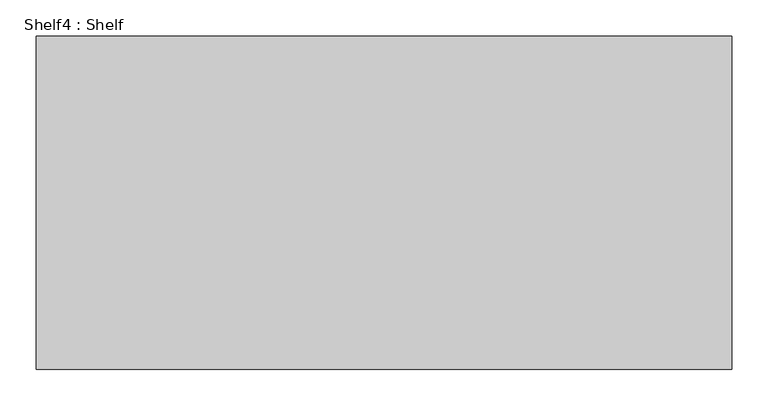
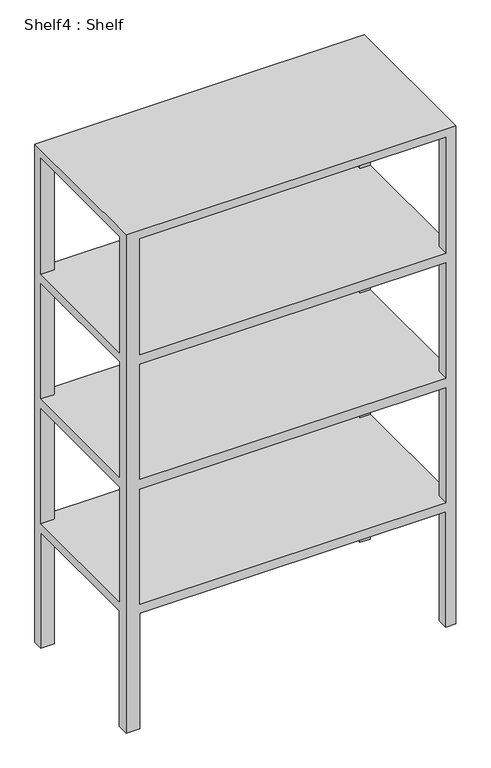
"""IFC4 building model written with IfcOpenShell, lengths in millimetres: furniture geometry, Shelf4 : Shelf."""

from ifc_helpers import new_model, si_unit, origin, place, context, project, spatial, faceted_brep, source, transform, mapped, element, save


def shelf4_shelf_8ff96b21(model_context):
    return source(origin(), model_context, "Body", "Brep", [
        faceted_brep([(14056.7001442, 2274.5615366, 1524.0), (14056.7001442, 2731.7615366, 1524.0), (13103.4798744, 2731.7615366, 1524.0), (13103.4798744, 2274.5615366, 1524.0), (14056.7001442, 2274.5615366, 0.0), (14028.3529362, 2274.5615366, 0.0), (14028.3529362, 2307.1181796, 0.0), (14056.7001442, 2307.1181796, 0.0), (14027.0281946, 2731.7615366, 0.0), (14056.7001442, 2731.7615366, 0.0), (14056.7001442, 2702.8377422, 0.0), (14027.0281946, 2702.8377422, 0.0), (13142.3001442, 2274.5615366, 0.0), (13103.4798744, 2274.5615366, 0.0), (13103.4798744, 2308.3555128, 0.0), (13142.3001442, 2308.3555128, 0.0), (13103.4798744, 2702.8377422, 0.0), (13103.4798744, 2731.7615366, 0.0), (13142.3001442, 2731.7615366, 0.0), (13142.3001442, 2702.8377422, 0.0), (13142.3001442, 2274.5615366, 353.3332002), (14028.3529362, 2274.5615366, 353.3332002), (13142.3001442, 2274.5615366, 1497.6781444), (14028.3529362, 2274.5615366, 1497.6781444), (14028.3529362, 2274.5615366, 1143.0), (13142.3001442, 2274.5615366, 1143.0), (13142.3001442, 2274.5615366, 1114.8196695), (14028.3529362, 2274.5615366, 1114.8196695), (14028.3529362, 2274.5615366, 762.0), (13142.3001442, 2274.5615366, 762.0), (13142.3001442, 2274.5615366, 731.9611947), (14028.3529362, 2274.5615366, 731.9611947), (14028.3529362, 2274.5615366, 381.0), (13142.3001442, 2274.5615366, 381.0), (13103.4798744, 2702.8377422, 353.3332002), (13103.4798744, 2308.3555128, 353.3332002), (13103.4798744, 2702.8377422, 1497.6781444), (13103.4798744, 2308.3555128, 1497.6781444), (13103.4798744, 2308.3555128, 1143.0), (13103.4798744, 2702.8377422, 1143.0), (13103.4798744, 2702.8377422, 1114.8196695), (13103.4798744, 2308.3555128, 1114.8196695), (13103.4798744, 2308.3555128, 762.0), (13103.4798744, 2702.8377422, 762.0), (13103.4798744, 2702.8377422, 731.9611947), (13103.4798744, 2308.3555128, 731.9611947), (13103.4798744, 2308.3555128, 381.0), (13103.4798744, 2702.8377422, 381.0), (14027.0281946, 2731.7615366, 353.3332002), (13142.3001442, 2731.7615366, 353.3332002), (14027.0281946, 2731.7615366, 1497.6781444), (13142.3001442, 2731.7615366, 1497.6781444), (13142.3001442, 2731.7615366, 1143.0), (14027.0281946, 2731.7615366, 1143.0), (14027.0281946, 2731.7615366, 1114.8196695), (13142.3001442, 2731.7615366, 1114.8196695), (13142.3001442, 2731.7615366, 762.0), (14027.0281946, 2731.7615366, 762.0), (14027.0281946, 2731.7615366, 731.9611947), (13142.3001442, 2731.7615366, 731.9611947), (13142.3001442, 2731.7615366, 381.0), (14027.0281946, 2731.7615366, 381.0), (14056.7001442, 2307.1181796, 353.3332002), (14056.7001442, 2702.8377422, 353.3332002), (14056.7001442, 2307.1181796, 1497.6781444), (14056.7001442, 2702.8377422, 1497.6781444), (14056.7001442, 2702.8377422, 1143.0), (14056.7001442, 2307.1181796, 1143.0), (14056.7001442, 2307.1181796, 1114.8196695), (14056.7001442, 2702.8377422, 1114.8196695), (14056.7001442, 2702.8377422, 762.0), (14056.7001442, 2307.1181796, 762.0), (14056.7001442, 2307.1181796, 731.9611947), (14056.7001442, 2702.8377422, 731.9611947), (14056.7001442, 2702.8377422, 381.0), (14056.7001442, 2307.1181796, 381.0), (13142.3001442, 2702.8377422, 1497.6781444), (14027.0281946, 2702.8377422, 1497.6781444), (14028.3529362, 2307.1181796, 1497.6781444), (13142.3001442, 2308.3555128, 1497.6781444), (13142.3001442, 2702.8377422, 1143.0), (13142.3001442, 2308.3555128, 1143.0), (14028.3529362, 2307.1181796, 1143.0), (14027.0281946, 2702.8377422, 1143.0), (13142.3001442, 2702.8377422, 1114.8196695), (14027.0281946, 2702.8377422, 1114.8196695), (14028.3529362, 2307.1181796, 1114.8196695), (13142.3001442, 2308.3555128, 1114.8196695), (13142.3001442, 2702.8377422, 762.0), (13142.3001442, 2308.3555128, 762.0), (14028.3529362, 2307.1181796, 762.0), (14027.0281946, 2702.8377422, 762.0), (13142.3001442, 2702.8377422, 731.9611947), (14027.0281946, 2702.8377422, 731.9611947), (14028.3529362, 2307.1181796, 731.9611947), (13142.3001442, 2308.3555128, 731.9611947), (13142.3001442, 2702.8377422, 381.0), (13142.3001442, 2308.3555128, 381.0), (14028.3529362, 2307.1181796, 381.0), (14027.0281946, 2702.8377422, 381.0), (13142.3001442, 2702.8377422, 353.3332002), (14027.0281946, 2702.8377422, 353.3332002), (14028.3529362, 2307.1181796, 353.3332002), (13142.3001442, 2308.3555128, 353.3332002)], [[[0, 1, 2, 3]], [[4, 5, 6, 7]], [[8, 9, 10, 11]], [[12, 13, 14, 15]], [[16, 17, 18, 19]], [[0, 3, 13, 12, 20, 21, 5, 4], [22, 23, 24, 25], [26, 27, 28, 29], [30, 31, 32, 33]], [[3, 2, 17, 16, 34, 35, 14, 13], [36, 37, 38, 39], [40, 41, 42, 43], [44, 45, 46, 47]], [[2, 1, 9, 8, 48, 49, 18, 17], [50, 51, 52, 53], [54, 55, 56, 57], [58, 59, 60, 61]], [[1, 0, 4, 7, 62, 63, 10, 9], [64, 65, 66, 67], [68, 69, 70, 71], [72, 73, 74, 75]], [[76, 51, 50, 77, 65, 64, 78, 23, 22, 79, 37, 36]], [[80, 39, 38, 81, 25, 24, 82, 67, 66, 83, 53, 52]], [[51, 76, 80, 52]], [[77, 50, 53, 83]], [[65, 77, 83, 66]], [[78, 64, 67, 82]], [[23, 78, 82, 24]], [[79, 22, 25, 81]], [[37, 79, 81, 38]], [[76, 36, 39, 80]], [[84, 55, 54, 85, 69, 68, 86, 27, 26, 87, 41, 40]], [[88, 43, 42, 89, 29, 28, 90, 71, 70, 91, 57, 56]], [[55, 84, 88, 56]], [[85, 54, 57, 91]], [[69, 85, 91, 70]], [[86, 68, 71, 90]], [[27, 86, 90, 28]], [[87, 26, 29, 89]], [[41, 87, 89, 42]], [[84, 40, 43, 88]], [[92, 59, 58, 93, 73, 72, 94, 31, 30, 95, 45, 44]], [[96, 47, 46, 97, 33, 32, 98, 75, 74, 99, 61, 60]], [[59, 92, 96, 60]], [[93, 58, 61, 99]], [[73, 93, 99, 74]], [[94, 72, 75, 98]], [[31, 94, 98, 32]], [[95, 30, 33, 97]], [[45, 95, 97, 46]], [[92, 44, 47, 96]], [[100, 49, 48, 101, 63, 62, 102, 21, 20, 103, 35, 34]], [[49, 100, 19, 18]], [[101, 48, 8, 11]], [[63, 101, 11, 10]], [[102, 62, 7, 6]], [[21, 102, 6, 5]], [[103, 20, 12, 15]], [[35, 103, 15, 14]], [[100, 34, 16, 19]]]),
    ])


if __name__ == "__main__":
    model = new_model("IFC4")
    model_context = context("Model", 3, world=origin())
    ifc_project = project(units=[si_unit("LENGTHUNIT", "METRE", prefix="MILLI")], contexts=[model_context])
    site = spatial("IfcSite", under=ifc_project)
    building = spatial("IfcBuilding", under=site)
    placement = place(None, origin())
    shelf4_shelf_shape = shelf4_shelf_8ff96b21(model_context)
    element("IfcFurniture", 1, ObjectType="Shelf4 : Shelf", at=placement, inside=building, context=model_context, shape_type="MappedRepresentation", body=[
        mapped(shelf4_shelf_shape, transform((0.0, 0.0, 0.0), x_axis=(1.0, 0.0, 0.0), y_axis=(0.0, 1.0, 0.0), z_axis=(0.0, 0.0, 1.0))),
    ])
    save(model, "model.ifc")

# Revit data of these elements
# Element 1 (IfcFurniture, "Shelf4 : Shelf")
#   Materials on its faces: "food"
# Materials
#   "food": class "Glass", colour RGB 233 233 233, transparency 0, Description = "Soda Lime Glass", Cost = 0
